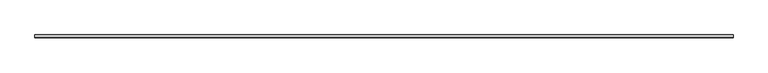
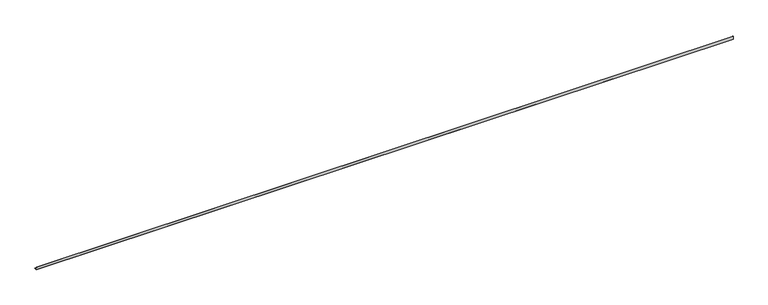
"""IFC4 building model written with IfcOpenShell, lengths in millimetres: proxy geometry, Generic Models 7:Generic Models 1:2:Generic Models 1:2 : Generic Models 7:Generic Models 1:337419:29 : Generic Models 7:Generic Models 1:2:Generic Models 1:2 : Generic Models 7:Generic Models 1:337419:306751."""

from ifc_helpers import new_model, si_unit, frame, origin, place, context, project, spatial, polyline, outline, extrude, source, transform, mapped, element, save


def generic_models_c4c7e4a8(model_context):
    return source(origin(), model_context, "Body", "SweptSolid", [
        extrude(outline(polyline([(-579006.609007, 3600.1736708), (-579006.609007, 3598.5861708), (-579007.402757, 3598.5861708), (-579007.402757, 3619.2236708), (-579006.609007, 3619.2236708), (-579006.609007, 3600.9674208), (-578988.352757, 3600.9674208), (-578988.352757, 3600.1736708), (-579006.609007, 3600.1736708)])), frame((591306.0367239, 0.0, 0.0), z_axis=(1.0, 0.0, 0.0), x_axis=(0.0, 1.0, 0.0)), (0.0, 0.0, 1.0), 4876.8),
    ])


if __name__ == "__main__":
    model = new_model("IFC4")
    model_context = context("Model", 3, world=origin())
    ifc_project = project(units=[si_unit("LENGTHUNIT", "METRE", prefix="MILLI")], contexts=[model_context])
    site = spatial("IfcSite", under=ifc_project)
    building = spatial("IfcBuilding", under=site)
    placement = place(None, origin())
    generic_models_shape = generic_models_c4c7e4a8(model_context)
    element("IfcBuildingElementProxy", 1, Name="Generic Models 7:Generic Models 1:2:Generic Models 1:2 : Generic Models 7:Generic Models 1:337419:29 : Generic Models 7:Generic Models 1:2:Generic Models 1:2 : Generic Models 7:Generic Models 1:337419:306751", ObjectType="Generic Models 7:Generic Models 1:2:Generic Models 1:2 : Generic Models 7:Generic Models 1:337419:29 : Generic Models 7:Generic Models 1:2:Generic Models 1:2 : Generic Models 7:Generic Models 1:337419:306751", at=placement, inside=building, context=model_context, shape_type="MappedRepresentation", body=[
        mapped(generic_models_shape, transform((0.0, 0.0, 0.0), x_axis=(1.0, 0.0, 0.0), y_axis=(0.0, 1.0, 0.0), z_axis=(0.0, 0.0, 1.0))),
    ])
    save(model, "model.ifc")

# Revit data of these elements
# Type "Generic Models 7:Generic Models 1:2:Generic Models 1:2 : Generic Models 7:Generic Models 1:337419:29 : Generic Models 7:Generic Models 1:2:Generic Models 1:2 : Generic Models 7:Generic Models 1:337419:306751"
#   NameOverride = "Generic Models 7:Generic Models 1:2:Generic Models 1:2 : Generic Models 7:Generic Models 1:337419:306751"
#   ObjectTypeOverride = "Generic Models 1:2 : Generic Models 7:Generic Models 1:337419"
#   Reference = "Generic Models 1"
#   Tag = "306751"
# Element 1 (IfcBuildingElementProxy, "Generic Models 7:Generic Models 1:2:Generic Models 1:2 : Generic Models 7:Generic Models 1:337419:29 : Generic Models 7:Generic Models 1:2:Generic Models 1:2 : Generic Models 7:Generic Models 1:337419:306751")
#   Materials on its faces: "J BEAD"
# Materials
#   "J BEAD": class "Generic", colour RGB 120 120 120, transparency 0, Cost = 0
